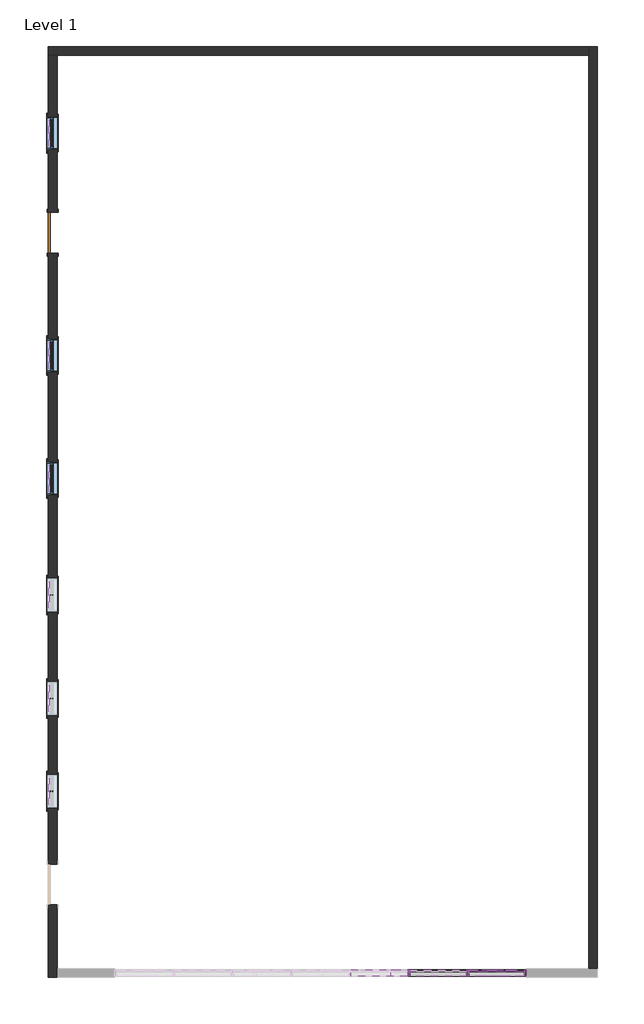
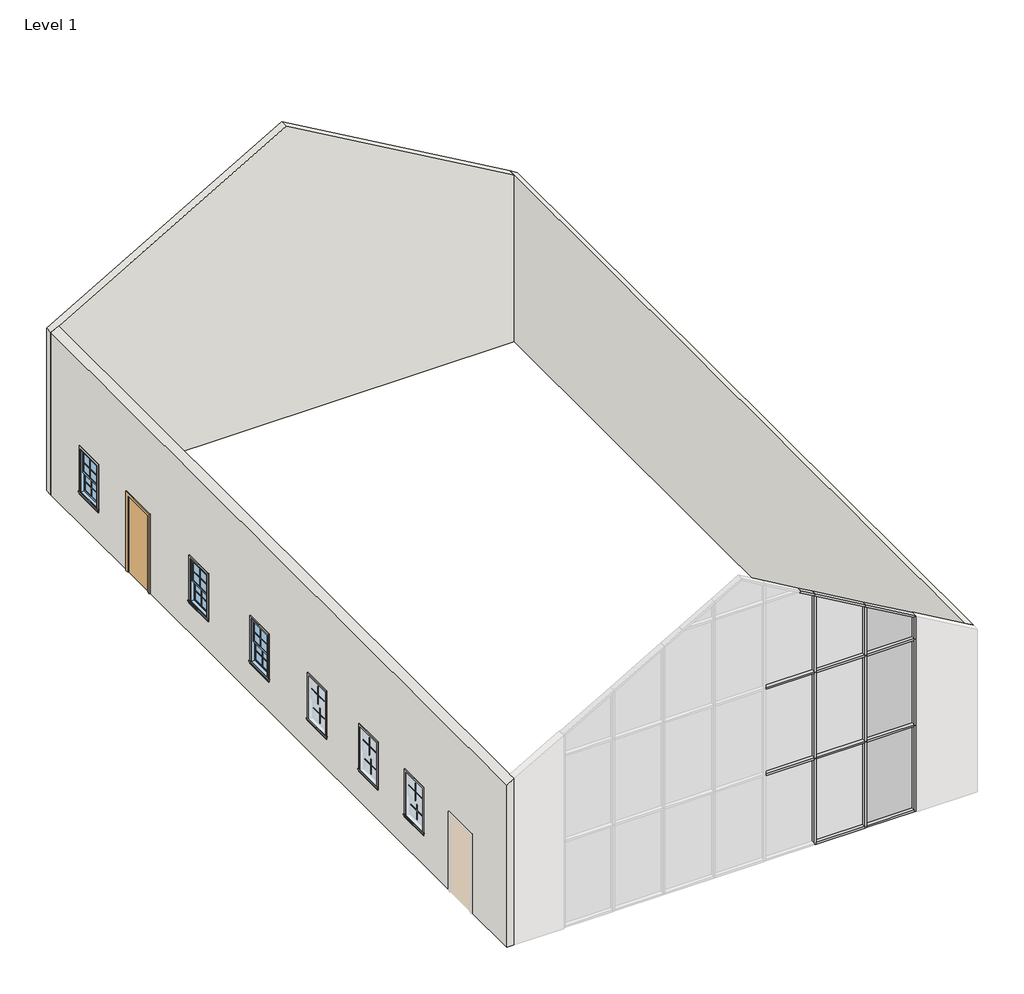
# One storey, part 2 of 2: 24 proxies, 20 members, 3 plates, 3 walls, 3 windows, 1 door.
# Revit data of these elements (continued)
# Element 54 (IfcWindow, "M_Window-Double-Hung : 750 x 1200mm") (continued)
#   Frame Extension = 31.75 mm
#   Exterior Wall Closure = 12.7 mm
#   Interior Trim Visibility = yes
#   Indicator Visibility = yes
#   Exterior Trim Visibility = yes
#   Phase Created = New Construction
#   Materials on its faces: "Wood - Stained", "Glass", "Clad - White"
# Materials
#   "Door - Panel": class "Wood", colour RGB 210 159 95, transparency 0, Cost = 0
#   "Door - Frame": class "Miscellaneous", colour RGB 118 70 51, transparency 0, Cost = 0
#   "Wood - Stained": class "Wood", colour RGB 227 170 128, transparency 0, Cost = 0
#   "Clad - White": class "Wood", colour RGB 242 242 238, transparency 0, Cost = 0
#   "Glass": class "Glass", colour RGB 0 128 192, transparency 0.75, Description = "Soda Lime Glass", Cost = 0
#   "Aluminum": class "Metal", colour RGB 247 247 247, transparency 0, Description = "Aluminum 6061", Cost = 0
#   "Default Wall": class "Miscellaneous", colour RGB 128 128 128, transparency 0, Cost = 0
